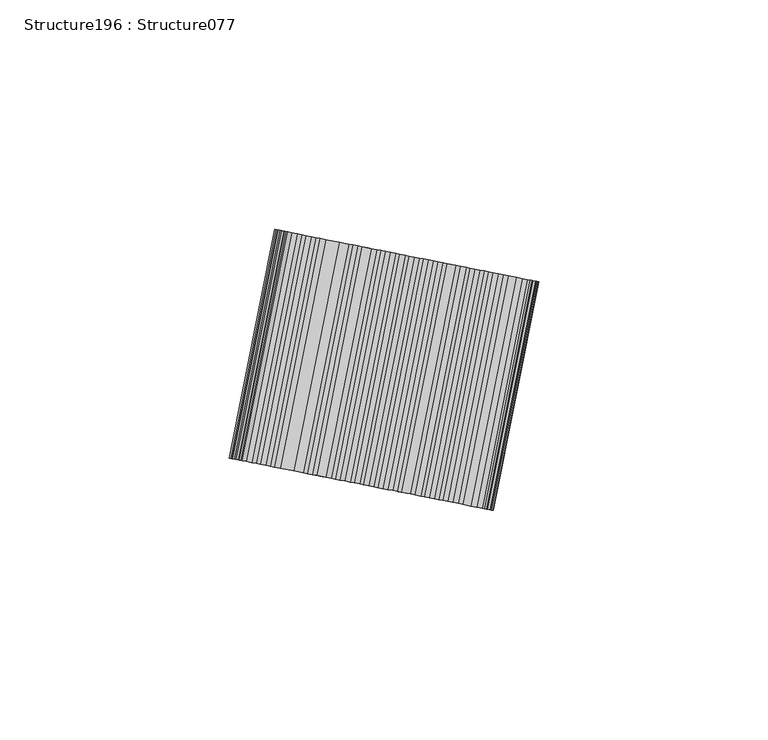
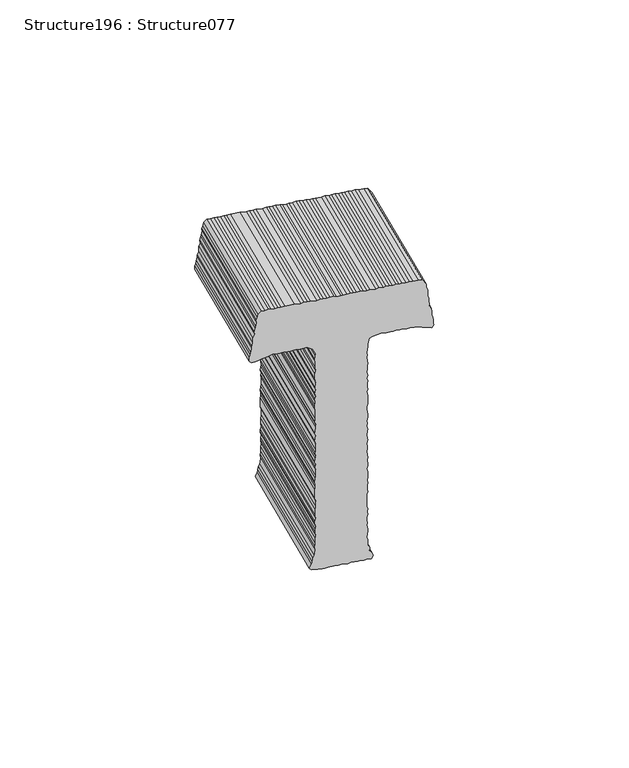
"""IFC4 building model written with IfcOpenShell, lengths in millimetres: proxy geometry, Structure196 : Structure077."""

from ifc_helpers import new_model, si_unit, frame, origin, place, context, project, spatial, polyline, outline, extrude, source, transform, mapped, element, save


def structure196_structure077_09110ab6(model_context):
    return source(origin(), model_context, "Body", "SweptSolid", [
        extrude(outline(polyline([(1.289959, 0.0), (2.4826397, -0.634609), (3.3164572, -1.0932808), (3.9580093, -1.9186696), (4.9710554, -2.555887), (5.615166, -3.0146846), (6.7250255, -3.5599983), (7.3660727, -4.3848856), (8.4728289, -4.7530823), (9.8531305, -6.1242605), (10.9554404, -6.6690959), (11.5100349, -7.2200247), (12.6129687, -7.9530557), (13.4427489, -8.4082185), (14.272529, -8.8633811), (15.1037896, -9.6891474), (15.1944421, -10.6985221), (14.1870201, -11.5298818), (13.2730324, -12.0849253), (12.3559164, -12.4553038), (11.5300276, -13.097864), (10.7973441, -13.4709018), (9.049314, -14.4858702), (8.3217174, -15.4066268), (7.7726497, -16.1431227), (6.9457746, -16.7917246), (6.1253802, -17.8013525), (5.4844271, -18.4465703), (4.5633947, -19.0016371), (3.7416407, -19.8288587), (3.2853708, -20.4764834), (2.2751721, -21.3050847), (1.5439439, -22.0411781), (1.0973356, -24.1608889), (1.6488975, -25.9977611), (2.4780177, -26.6333239), (3.3998042, -27.3679621), (4.0491583, -28.1940798), (5.430722, -29.5665119), (6.2585694, -30.5769647), (7.1799825, -31.1231547), (8.4699131, -32.4045594), (9.2069822, -33.5058896), (10.7732057, -34.8736837), (11.2367929, -35.5222839), (12.2485769, -36.1582475), (12.8912362, -37.1657919), (13.6346843, -37.5351933), (14.4614986, -38.5375983), (15.2886228, -39.1781998), (15.9366173, -39.8219113), (16.6745753, -40.7360473), (18.7947567, -42.8422151), (19.7140188, -43.5743456), (20.1741694, -44.4005875), (21.0044202, -45.2253507), (22.6654609, -46.5062796), (23.0352406, -47.2427481), (24.6922423, -48.5196648), (25.2470551, -49.4399433), (26.8111275, -50.9936778), (27.6447916, -51.6337544), (28.4723865, -52.6439565), (29.1169786, -53.0962108), (30.038765, -53.8308488), (30.5895388, -54.7471151), (31.332832, -55.2974182), (31.9756463, -56.1240609), (33.5424955, -57.6805538), (34.2814973, -58.2265939), (35.2908778, -59.0482471), (35.8480941, -59.782836), (36.4905351, -60.4210307), (37.3206885, -61.0646414), (39.6269128, -63.3556224), (40.0845389, -64.1793567), (41.5610173, -65.646076), (42.5766853, -66.4669536), (43.9585014, -67.8396365), (44.6000534, -68.6650253), (45.5239909, -69.213723), (46.1692087, -69.8546761), (46.7214971, -70.7724469), (47.6467942, -71.5035509), (48.3821304, -72.2340269), (49.0277214, -73.0634279), (49.9502418, -73.7917736), (51.2404248, -75.073429), (52.0662869, -75.7127767), (52.8989071, -76.7209493), (54.5549225, -78.0039076), (55.4788925, -78.1830032), (56.4913023, -79.0076656), (57.2264202, -79.3687917), (58.6082305, -79.8291689), (58.7026461, -80.8352603), (57.9676564, -81.5751403), (57.3267991, -82.4010074), (56.50542, -83.4171802), (55.9549927, -83.9712698), (55.1291023, -84.6133267), (53.6628845, -86.0893002), (52.935542, -87.0108108), (52.1058901, -87.6566542), (51.2838853, -88.4841283), (50.7378453, -89.2231302), (49.9083484, -89.6880719), (49.1771202, -90.4241654), (48.4419756, -91.3449471), (47.7141623, -91.8968573), (47.1679672, -92.8167608), (46.0633821, -93.5586212), (45.4222741, -94.3847406), (44.2272873, -94.1169737), (43.8574102, -93.1993528), (43.5804608, -92.0044109), (42.6585769, -91.0886204), (42.5601223, -90.0785167), (40.9893892, -88.3371098), (40.6233961, -87.6044028), (39.7960195, -86.9635506), (38.8722369, -86.2339511), (38.2270192, -85.5929981), (37.4927269, -84.4944262), (36.8448298, -84.0318672), (36.0162486, -83.0277069), (35.3672443, -82.3829923), (34.4470933, -81.8380562), (33.8989413, -81.1054499), (33.0652771, -80.4653733), (32.5145034, -79.549107), (29.3755039, -76.4308552), (28.6416481, -76.0709829), (27.9988339, -75.2443401), (27.0731636, -74.3247881), (26.2422762, -73.6874699), (25.6009766, -72.8623318), (24.9520931, -72.4058145), (23.3854963, -70.8495724), (22.7428371, -69.8420279), (21.8214239, -69.295838), (21.1736818, -68.6523772), (20.5308676, -67.8257344), (19.6096093, -67.0986427), (18.3179459, -65.4463837), (17.5794256, -64.8938004), (16.7509417, -64.0707925), (16.2921742, -63.4340016), (15.0900559, -62.6089619), (14.6310127, -61.9648754), (13.9887267, -61.1457791), (12.9725305, -60.3173552), (12.3279383, -59.8651009), (11.6784635, -58.8507858), (10.945749, -58.30397), (10.2991717, -57.4806107), (9.2805719, -56.8378765), (8.4536027, -56.0163732), (7.9067128, -55.2850208), (7.2560966, -54.4576492), (6.6108788, -53.8166961), (5.6869413, -53.2679985), (3.4748743, -51.0705525), (2.740582, -49.9719806), (1.9113067, -49.5173195), (1.3560867, -48.7776919), (0.620498, -48.0469653), (-0.2129137, -47.4071395), (-0.7654545, -46.4891177), (-1.6823239, -45.9474415), (-2.3317988, -44.9331264), (-3.1594278, -44.2920234), (-3.8950165, -43.5612967), (-4.8203136, -42.8301928), (-6.1079382, -41.181946), (-6.9378391, -40.538586), (-7.3981213, -39.9002905), (-8.3199077, -39.1656524), (-9.1505426, -38.5285851), (-9.7955079, -37.8878827), (-11.5384177, -36.8807157), (-12.461183, -37.0649281), (-13.8384529, -37.8980173), (-14.8461289, -38.7286231), (-15.3965562, -39.2827127), (-16.0358989, -40.1100843), (-16.9497891, -40.8462803), (-17.5928933, -41.6774384), (-18.6009409, -42.3200993), (-19.0556004, -43.1498778), (-19.8825963, -43.6102824), (-20.612344, -44.7169794), (-21.3486933, -45.2744531), (-23.1741728, -47.6684523), (-23.7231446, -48.5855975), (-24.1776816, -49.6040764), (-24.6342273, -50.2444055), (-25.1856026, -51.3472402), (-26.2867063, -51.1662161), (-26.7507748, -50.5241592), (-27.5782489, -49.7021544), (-28.1285195, -48.7858863), (-28.5969769, -47.9584139), (-29.4239461, -47.1369107), (-30.1573836, -46.2202437), (-30.4442845, -45.2110165), (-30.9911744, -44.4796641), (-31.5499052, -43.7435707), (-32.286756, -43.0115902), (-32.7467531, -42.0039433), (-33.6726759, -41.0841405), (-34.3148645, -40.4461966), (-34.684839, -39.3474232), (-35.5160996, -38.521657), (-35.9848061, -36.4049811), (-35.1593865, -35.3933237), (-33.877731, -34.1031406), (-33.2381376, -33.2755166), (-32.3207367, -32.5357866), (-31.5906173, -31.6170343), (-30.7675037, -30.972219), (-30.2149253, -30.2321891), (-29.3014408, -29.6771472), (-28.7522182, -28.7597497), (-27.9267027, -27.9287415), (-27.1977806, -27.5594901), (-26.460485, -26.4527681), (-25.5467496, -25.8974738), (-24.2649393, -24.426389), (-23.533866, -23.8711972), (-22.7988765, -23.1313173), (-22.2496538, -22.2139197), (-21.3360144, -21.4779761), (-20.6929102, -20.6468181), (-20.0522079, -20.0018527), (-19.1383176, -19.2656567), (-18.3128022, -18.4346486), (-17.6722547, -17.970585), (-16.7597242, -17.0519828), (-16.3880426, -16.3133075), (-15.4757627, -15.3949576), (-14.6488876, -14.7463557), (-14.0092941, -13.9187317), (-13.3685918, -13.2737664), (-12.3608199, -12.6238099), (-11.0803692, -10.9703188), (-10.3440199, -10.4128451), (-9.6141514, -9.4943454), (-8.7909419, -9.0301793), (-7.5104912, -7.3766882), (-5.3998096, -5.2519629), (-4.3918828, -4.4211047), (-3.7546912, -3.7796735), (-2.9293306, -3.1295671), (-2.1976967, -2.2123194), (-1.6488799, -1.476076), (-0.7316339, -0.9172477), (0.0, 0.0), (1.289959, 0.0)])), frame((-2585.4799939, 234981.5888059, 485.405184), z_axis=(0.1946622229639412, 0.9808703374813293, 0.0), x_axis=(-0.6912765086622871, 0.13718981675446087, -0.7094474911863151)), (0.0, 0.0, 1.0), 50.8),
    ])


if __name__ == "__main__":
    model = new_model("IFC4")
    model_context = context("Model", 3, world=origin())
    ifc_project = project(units=[si_unit("LENGTHUNIT", "METRE", prefix="MILLI")], contexts=[model_context])
    site = spatial("IfcSite", under=ifc_project)
    building = spatial("IfcBuilding", under=site)
    placement = place(None, origin())
    structure196_structure077_shape = structure196_structure077_09110ab6(model_context)
    element("IfcBuildingElementProxy", 1, Name="Structure196 : Structure077", ObjectType="Structure196 : Structure077", at=placement, inside=building, context=model_context, shape_type="MappedRepresentation", body=[
        mapped(structure196_structure077_shape, transform((0.0, 0.0, 0.0), x_axis=(1.0, 0.0, 0.0), y_axis=(0.0, 1.0, 0.0), z_axis=(0.0, 0.0, 1.0))),
    ])
    save(model, "model.ifc")

# Revit data of these elements
# Type "Structure196 : Structure077"
#   NameOverride = "Structure077"
# Element 1 (IfcBuildingElementProxy, "Structure196 : Structure077")
#   Materials on its faces: "BRUSHED ALUMINUM LETTERING"
# Materials
#   "BRUSHED ALUMINUM LETTERING": class "Unassigned", colour RGB 169 181 186, transparency 0, Cost = 0
